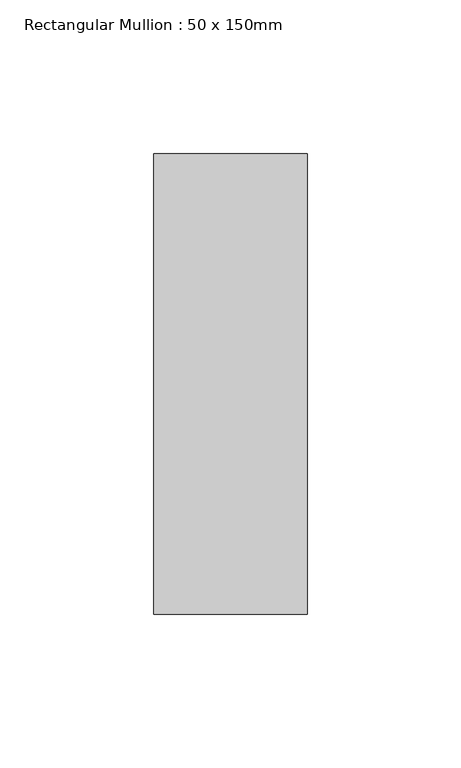
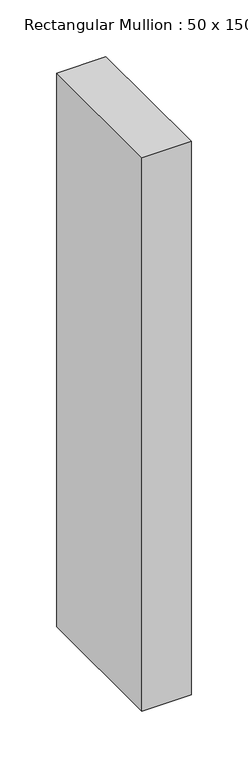
"""IFC4 building model written with IfcOpenShell, lengths in millimetres: member geometry, Rectangular Mullion : 50 x 150mm."""

from ifc_helpers import new_model, si_unit, frame, origin, place, context, project, spatial, polyline, outline, extrude, source, transform, mapped, element, save


def rectangular_mullion_50_x_150mm_431ffd9c(model_context):
    return source(origin(), model_context, "Body", "SweptSolid", [
        extrude(outline(polyline([(25.0, 75.0), (25.0, -75.0), (-25.0, -75.0), (-25.0, 75.0), (25.0, 75.0)])), frame((0.0, 0.0, -595.0), z_axis=(0.0, 0.0, 1.0), x_axis=(1.0, 0.0, 0.0)), (0.0, 0.0, 1.0), 595.0),
    ])


if __name__ == "__main__":
    model = new_model("IFC4")
    model_context = context("Model", 3, world=origin())
    ifc_project = project(units=[si_unit("LENGTHUNIT", "METRE", prefix="MILLI")], contexts=[model_context])
    site = spatial("IfcSite", under=ifc_project)
    building = spatial("IfcBuilding", under=site)
    placement = place(None, origin())
    rectangular_mullion_50_x_150mm_shape = rectangular_mullion_50_x_150mm_431ffd9c(model_context)
    element("IfcMember", 1, ObjectType="Rectangular Mullion : 50 x 150mm", at=placement, inside=building, context=model_context, shape_type="MappedRepresentation", body=[
        mapped(rectangular_mullion_50_x_150mm_shape, transform((0.0, 0.0, 0.0), x_axis=(1.0, 0.0, 0.0), y_axis=(0.0, 1.0, 0.0), z_axis=(0.0, 0.0, 1.0))),
    ])
    save(model, "model.ifc")

# Revit data of these elements
# Type "Rectangular Mullion : 50 x 150mm"
#   built-in parameter 1007304 = 0.492126 (stored number, unit not read)
#   built-in parameter 1007301 = 0.082021 (stored number, unit not read)
#   built-in parameter 1007300 = 0.082021 (stored number, unit not read)
# Element 1 (IfcMember, "Rectangular Mullion : 50 x 150mm")
#   Materials on its faces: "Metal - Aluminium"
# Materials
#   "Metal - Aluminium": class "Metal", colour RGB 247 247 247, transparency 0
